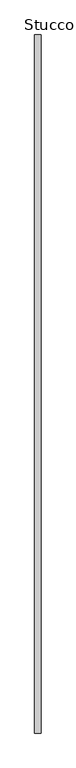
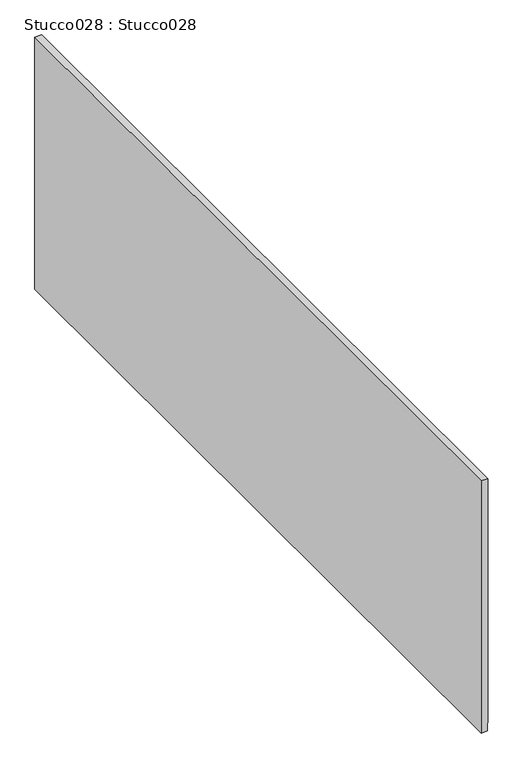
"""IFC4 building model written with IfcOpenShell, lengths in millimetres: proxy geometry, Stucco028 : Stucco028."""

from ifc_helpers import new_model, si_unit, frame, origin, place, context, project, spatial, polyline, outline, extrude, source, transform, mapped, element, save


def stucco028_stucco028_36482e62(model_context):
    return source(origin(), model_context, "Body", "SweptSolid", [
        extrude(outline(polyline([(39567.688258, -4377.698937), (40234.4061757, -4377.698937), (40234.4061757, -4395.4791416), (39545.1576447, -4395.4791416), (39545.1576447, -4378.9846986), (39567.688258, -4378.9846986), (39567.688258, -4377.698937)])), frame((0.0, -1065.3407312, 0.0), z_axis=(0.0, 1.0, 0.0), x_axis=(0.0, 0.0, 1.0)), (0.0, 0.0, 1.0), 2000.0),
    ])


if __name__ == "__main__":
    model = new_model("IFC4")
    model_context = context("Model", 3, world=origin())
    ifc_project = project(units=[si_unit("LENGTHUNIT", "METRE", prefix="MILLI")], contexts=[model_context])
    site = spatial("IfcSite", under=ifc_project)
    building = spatial("IfcBuilding", under=site)
    placement = place(None, origin())
    stucco028_stucco028_shape = stucco028_stucco028_36482e62(model_context)
    element("IfcBuildingElementProxy", 1, Name="Stucco028 : Stucco028", ObjectType="Stucco028 : Stucco028", at=placement, inside=building, context=model_context, shape_type="MappedRepresentation", body=[
        mapped(stucco028_stucco028_shape, transform((0.0, 0.0, 0.0), x_axis=(1.0, 0.0, 0.0), y_axis=(0.0, 1.0, 0.0), z_axis=(0.0, 0.0, 1.0))),
    ])
    save(model, "model.ifc")

# Revit data of these elements
# Type "Stucco028 : Stucco028"
#   NameOverride = "Stucco028"
# Element 1 (IfcBuildingElementProxy, "Stucco028 : Stucco028")
#   Materials on its faces: "7/8\" SMOOTH TROWEL EXTERIOR STUCCO"
# Materials
#   "7/8\" SMOOTH TROWEL EXTERIOR STUCCO": class "Unassigned", colour RGB 255 255 255, transparency 0, Cost = 0
